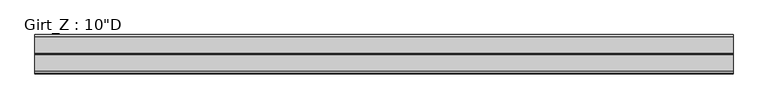
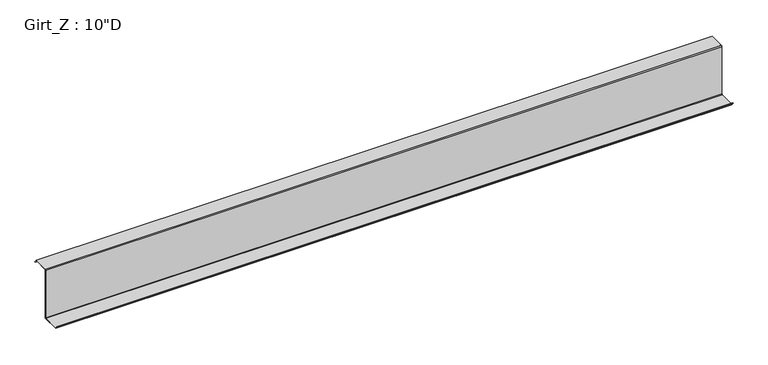
"""IFC4 building model written with IfcOpenShell, lengths in millimetres: beam geometry."""

from ifc_helpers import new_model, si_unit, point, frame, frame_2d, origin, place, context, project, spatial, polyline, circle_curve, trimmed, segment, composite_curve, outline, extrude, source, transform, mapped, element, save


def beam_b090a1c8(model_context):
    return source(origin(), model_context, "Body", "SweptSolid", [
        extrude(outline(composite_curve([segment(polyline([(77.9859375, 127.0), (90.2310415, 112.4068534), (88.1028742, 110.621109), (76.6904765, 124.221875), (3.3005807, 124.221875)]), True, "CONTINUOUS"), segment(trimmed(circle_curve(frame_2d((3.3741066, 122.2381931)), 1.9850441), [point((3.3005807, 124.221875))], [point((1.3890625, 122.2381931))], True, "CARTESIAN"), True, "CONTINUOUS"), segment(polyline([(1.3890625, 122.2381931), (1.3890625, -127.0), (-84.3359375, -127.0), (-96.5810415, -112.4068534), (-94.4528742, -110.621109), (-83.0404765, -124.221875), (-3.2694106, -124.221875)]), True, "CONTINUOUS"), segment(trimmed(circle_curve(frame_2d((-3.3748024, -122.2389339)), 1.9857399), [point((-3.2694106, -124.221875))], [point((-1.3890625, -122.2389339))], True, "CARTESIAN"), True, "CONTINUOUS"), segment(polyline([(-1.3890625, -122.2389339), (-1.3890625, 122.2375)]), True, "CONTINUOUS"), segment(trimmed(circle_curve(frame_2d((3.3734375, 122.2375)), 4.7625), [point((-1.3890625, 122.2375))], [point((3.3734375, 127.0))], False, "CARTESIAN"), True, "CONTINUOUS"), segment(polyline([(3.3734375, 127.0), (77.9859375, 127.0)]), True, "CONTINUOUS")], self_intersect=False)), frame((-1694.19383, 0.0, 0.0), z_axis=(1.0, 0.0, 0.0), x_axis=(0.0, 1.0, 0.0)), (0.0, 0.0, 1.0), 3302.28166),
    ])


if __name__ == "__main__":
    model = new_model("IFC4")
    model_context = context("Model", 3, world=origin())
    ifc_project = project(units=[si_unit("LENGTHUNIT", "METRE", prefix="MILLI")], contexts=[model_context])
    site = spatial("IfcSite", under=ifc_project)
    building = spatial("IfcBuilding", under=site)
    placement = place(None, origin())
    beam_shape = beam_b090a1c8(model_context)
    element("IfcBeam", 1, ObjectType="Girt_Z : 10\"D", at=placement, inside=building, context=model_context, shape_type="MappedRepresentation", body=[
        mapped(beam_shape, transform((0.0, 0.0, 0.0), x_axis=(1.0, 0.0, 0.0), y_axis=(0.0, 1.0, 0.0), z_axis=(0.0, 0.0, 1.0))),
    ])
    save(model, "model.ifc")

# Revit data of these elements
# Type "Girt_Z : 10\"D"
#   half leg = 0' - 1 11/16"
#   Web_Thickness = 0' - 0 7/64"
#   Length [instance default] = 10' - 0"
#   Leg_2 = 0' - 3 3/8"
#   Leg_1 = 0' - 3 1/8"
#   Height = 0' - 10"
#   Structural Material [instance default] = none
# Element 1 (IfcBeam, "Girt_Z : 10\"D")
#   Structural Material = STRUCTURAL STEEL - SEE STRUCT. DWGS
#   Materials on its faces: "STRUCTURAL STEEL - SEE STRUCT. DWGS"
# Materials
#   "STRUCTURAL STEEL - SEE STRUCT. DWGS": class "Metal", colour RGB 137 146 153, transparency 0, Description = "Steel, mill finish", Cost = 0
